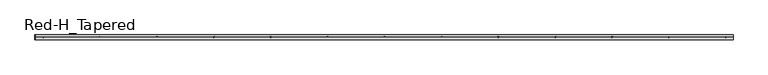
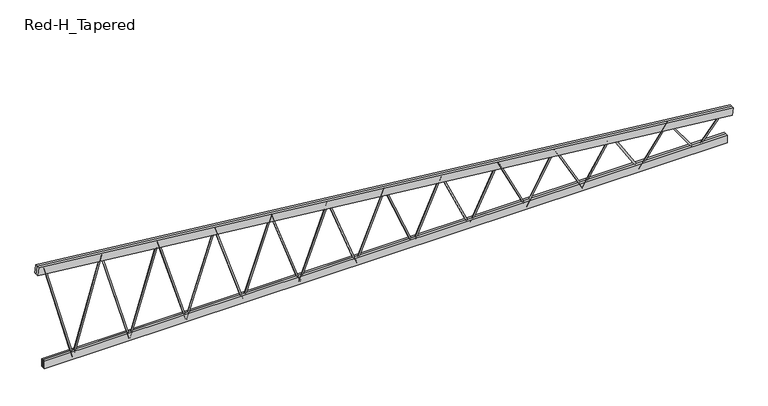
"""IFC4 building model written with IfcOpenShell, lengths in millimetres: beam geometry, Construction_Frames_RedBuilt_Openweb_Red-H_Tapered : Red-H_Tapered."""

from ifc_helpers import new_model, si_unit, point, frame, origin, origin_2d, place, context, project, spatial, polyline, circle_curve, trimmed, segment, composite_curve, outline, extrude, source, transform, mapped, element, save


def red_h_tapered_06906efe(model_context):
    return source(origin(), model_context, "Body", "SweptSolid", [
        extrude(outline(composite_curve([segment(trimmed(circle_curve(origin_2d(), 12.7), [point((0.0, -12.7))], [point((0.0, 12.7))], False, "CARTESIAN"), True, "CONTINUOUS"), segment(trimmed(circle_curve(origin_2d(), 12.7), [point((0.0, 12.7))], [point((0.0, -12.7))], False, "CARTESIAN"), True, "CONTINUOUS")], self_intersect=False)), frame((-491.6619792, 0.0, -367.0101562), z_axis=(-0.3557899484790522, 0.0, 0.9345659487490829), x_axis=(0.0, -1.0, 0.0)), (0.0, 0.0, 1.0), 1381.888334),
        extrude(outline(composite_curve([segment(trimmed(circle_curve(origin_2d(), 12.7), [point((0.0, 12.7))], [point((0.0, -12.6999999))], False, "CARTESIAN"), True, "CONTINUOUS"), segment(trimmed(circle_curve(origin_2d(), 12.7), [point((0.0, -12.6999999))], [point((0.0, 12.7))], False, "CARTESIAN"), True, "CONTINUOUS")], self_intersect=False)), frame((-1474.9859375, 0.0, -367.0101562), z_axis=(0.35578994847905304, 0.0, 0.9345659487490826), x_axis=(0.0, -1.0, 0.0)), (0.0, 0.0, 1.0), 1381.888334),
        extrude(outline(composite_curve([segment(trimmed(circle_curve(origin_2d(), 12.7), [point((0.0, -12.7))], [point((0.0, 12.6999999))], False, "CARTESIAN"), True, "CONTINUOUS"), segment(trimmed(circle_curve(origin_2d(), 12.7), [point((0.0, 12.6999999))], [point((0.0, -12.7))], False, "CARTESIAN"), True, "CONTINUOUS")], self_intersect=False)), frame((-1474.9859375, 0.0, -367.0101562), z_axis=(-0.33293456473962296, 0.0, 0.9429499327120385), x_axis=(0.0, -1.0, 0.0)), (0.0, 0.0, 1.0), 1476.7525852),
        extrude(outline(composite_curve([segment(trimmed(circle_curve(origin_2d(), 12.7), [point((0.0, -12.7))], [point((0.0, 12.7))], False, "CARTESIAN"), True, "CONTINUOUS"), segment(trimmed(circle_curve(origin_2d(), 12.7), [point((0.0, 12.7))], [point((0.0, -12.7))], False, "CARTESIAN"), True, "CONTINUOUS")], self_intersect=False)), frame((-2458.3098958, 0.0, -367.0101562), z_axis=(0.3329345647396264, 0.0, 0.9429499327120373), x_axis=(0.0, -1.0, 0.0)), (0.0, 0.0, 1.0), 1476.7525852),
        extrude(outline(composite_curve([segment(trimmed(circle_curve(origin_2d(), 12.7), [point((0.0, 12.7))], [point((0.0, -12.7))], False, "CARTESIAN"), True, "CONTINUOUS"), segment(trimmed(circle_curve(origin_2d(), 12.7), [point((0.0, -12.7))], [point((0.0, 12.7))], False, "CARTESIAN"), True, "CONTINUOUS")], self_intersect=False)), frame((-2458.3098958, 0.0, -367.0101562), z_axis=(-0.3126852540143423, 0.0, 0.9498567954812905), x_axis=(0.0, -1.0, 0.0)), (0.0, 0.0, 1.0), 1572.3862026),
        extrude(outline(composite_curve([segment(trimmed(circle_curve(origin_2d(), 12.7), [point((0.0, -12.7))], [point((0.0, 12.7))], False, "CARTESIAN"), True, "CONTINUOUS"), segment(trimmed(circle_curve(origin_2d(), 12.7), [point((0.0, 12.7))], [point((0.0, -12.7))], False, "CARTESIAN"), True, "CONTINUOUS")], self_intersect=False)), frame((-3441.6338542, 0.0, -367.0101562), z_axis=(0.31268525401434183, 0.0, 0.9498567954812908), x_axis=(0.0, -1.0, 0.0)), (0.0, 0.0, 1.0), 1572.3862026),
        extrude(outline(composite_curve([segment(trimmed(circle_curve(origin_2d(), 12.7), [point((0.0, 12.7))], [point((0.0, -12.7))], False, "CARTESIAN"), True, "CONTINUOUS"), segment(trimmed(circle_curve(origin_2d(), 12.7), [point((0.0, -12.7))], [point((0.0, 12.7))], False, "CARTESIAN"), True, "CONTINUOUS")], self_intersect=False)), frame((-3441.6338542, 0.0, -367.0101562), z_axis=(-0.29464533787098635, 0.0, 0.9556066789589179), x_axis=(0.0, -1.0, 0.0)), (0.0, 0.0, 1.0), 1668.6569104),
        extrude(outline(composite_curve([segment(trimmed(circle_curve(origin_2d(), 12.7), [point((0.0, -12.7))], [point((0.0, 12.7))], False, "CARTESIAN"), True, "CONTINUOUS"), segment(trimmed(circle_curve(origin_2d(), 12.7), [point((0.0, 12.7))], [point((0.0, -12.7))], False, "CARTESIAN"), True, "CONTINUOUS")], self_intersect=False)), frame((-4424.9578125, 0.0, -367.0101562), z_axis=(0.2946453378709914, 0.0, 0.9556066789589164), x_axis=(0.0, -1.0, 0.0)), (0.0, 0.0, 1.0), 1668.6569104),
        extrude(outline(composite_curve([segment(trimmed(circle_curve(origin_2d(), 12.7), [point((0.0, 12.7))], [point((0.0, -12.7))], False, "CARTESIAN"), True, "CONTINUOUS"), segment(trimmed(circle_curve(origin_2d(), 12.7), [point((0.0, -12.7))], [point((0.0, 12.7))], False, "CARTESIAN"), True, "CONTINUOUS")], self_intersect=False)), frame((-4424.9578125, 0.0, -367.0101562), z_axis=(-0.2784893697457471, 0.0, 0.9604393114292109), x_axis=(0.0, -1.0, 0.0)), (0.0, 0.0, 1.0), 1765.46049),
        extrude(outline(composite_curve([segment(trimmed(circle_curve(origin_2d(), 12.7), [point((0.0, -12.7))], [point((0.0, 12.6999999))], False, "CARTESIAN"), True, "CONTINUOUS"), segment(trimmed(circle_curve(origin_2d(), 12.7), [point((0.0, 12.6999999))], [point((0.0, -12.7))], False, "CARTESIAN"), True, "CONTINUOUS")], self_intersect=False)), frame((-5408.2817708, 0.0, -367.0101562), z_axis=(0.27848936974574684, 0.0, 0.9604393114292109), x_axis=(0.0, -1.0, 0.0)), (0.0, 0.0, 1.0), 1765.46049),
        extrude(outline(composite_curve([segment(trimmed(circle_curve(origin_2d(), 12.7), [point((0.0, 12.7))], [point((0.0, -12.7000001))], False, "CARTESIAN"), True, "CONTINUOUS"), segment(trimmed(circle_curve(origin_2d(), 12.7), [point((0.0, -12.7000001))], [point((0.0, 12.7))], False, "CARTESIAN"), True, "CONTINUOUS")], self_intersect=False)), frame((-5408.2817708, 0.0, -367.0101562), z_axis=(-0.2639492777400816, 0.0, 0.9645365616608265), x_axis=(0.0, -1.0, 0.0)), (0.0, 0.0, 1.0), 1862.7138645),
        extrude(outline(composite_curve([segment(trimmed(circle_curve(origin_2d(), 12.7), [point((0.0, 12.7000001))], [point((0.0, -12.6999999))], False, "CARTESIAN"), True, "CONTINUOUS"), segment(trimmed(circle_curve(origin_2d(), 12.7), [point((0.0, -12.6999999))], [point((0.0, 12.7000001))], False, "CARTESIAN"), True, "CONTINUOUS")], self_intersect=False)), frame((5408.2817708, 0.0, -367.0101562), z_axis=(0.6439089672678159, 0.0, 0.7651021120557013), x_axis=(0.0, -1.0, 0.0)), (0.0, 0.0, 1.0), 763.5582111),
        extrude(outline(composite_curve([segment(trimmed(circle_curve(origin_2d(), 12.7), [point((0.0, -12.7))], [point((0.0, 12.7))], False, "CARTESIAN"), True, "CONTINUOUS"), segment(trimmed(circle_curve(origin_2d(), 12.7), [point((0.0, 12.7))], [point((0.0, -12.7))], False, "CARTESIAN"), True, "CONTINUOUS")], self_intersect=False)), frame((5408.2817708, 0.0, -367.0101562), z_axis=(-0.5829691057722732, 0.0, 0.8124943210355849), x_axis=(0.0, -1.0, 0.0)), (0.0, 0.0, 1.0), 843.3757026),
        extrude(outline(composite_curve([segment(trimmed(circle_curve(origin_2d(), 12.7), [point((0.0, 12.7000001))], [point((0.0, -12.7))], False, "CARTESIAN"), True, "CONTINUOUS"), segment(trimmed(circle_curve(origin_2d(), 12.7), [point((0.0, -12.7))], [point((0.0, 12.7000001))], False, "CARTESIAN"), True, "CONTINUOUS")], self_intersect=False)), frame((4424.9578125, 0.0, -367.0101562), z_axis=(0.5829691057722711, 0.0, 0.8124943210355865), x_axis=(0.0, -1.0, 0.0)), (0.0, 0.0, 1.0), 843.3757026),
        extrude(outline(composite_curve([segment(trimmed(circle_curve(origin_2d(), 12.7), [point((0.0, -12.7))], [point((0.0, 12.6999999))], False, "CARTESIAN"), True, "CONTINUOUS"), segment(trimmed(circle_curve(origin_2d(), 12.7), [point((0.0, 12.6999999))], [point((0.0, -12.7))], False, "CARTESIAN"), True, "CONTINUOUS")], self_intersect=False)), frame((4424.9578125, 0.0, -367.0101562), z_axis=(-0.5301846601927273, 0.0, 0.8478822006011933), x_axis=(0.0, -1.0, 0.0)), (0.0, 0.0, 1.0), 927.3410117),
        extrude(outline(composite_curve([segment(trimmed(circle_curve(origin_2d(), 12.7), [point((0.0, 12.7))], [point((0.0, -12.7))], False, "CARTESIAN"), True, "CONTINUOUS"), segment(trimmed(circle_curve(origin_2d(), 12.7), [point((0.0, -12.7))], [point((0.0, 12.7))], False, "CARTESIAN"), True, "CONTINUOUS")], self_intersect=False)), frame((3441.6338542, 0.0, -367.0101562), z_axis=(0.5301846601927259, 0.0, 0.8478822006011942), x_axis=(0.0, -1.0, 0.0)), (0.0, 0.0, 1.0), 927.3410117),
        extrude(outline(composite_curve([segment(trimmed(circle_curve(origin_2d(), 12.7), [point((0.0, -12.7))], [point((0.0, 12.7))], False, "CARTESIAN"), True, "CONTINUOUS"), segment(trimmed(circle_curve(origin_2d(), 12.7), [point((0.0, 12.7))], [point((0.0, -12.7))], False, "CARTESIAN"), True, "CONTINUOUS")], self_intersect=False)), frame((3441.6338542, 0.0, -367.0101562), z_axis=(-0.48467074935534044, 0.0, 0.874696670120181), x_axis=(0.0, -1.0, 0.0)), (0.0, 0.0, 1.0), 1014.4246993),
        extrude(outline(composite_curve([segment(trimmed(circle_curve(origin_2d(), 12.7), [point((0.0, 12.7))], [point((0.0, -12.7))], False, "CARTESIAN"), True, "CONTINUOUS"), segment(trimmed(circle_curve(origin_2d(), 12.7), [point((0.0, -12.7))], [point((0.0, 12.7))], False, "CARTESIAN"), True, "CONTINUOUS")], self_intersect=False)), frame((2458.3098958, 0.0, -367.0101562), z_axis=(0.48467074935534116, 0.0, 0.8746966701201807), x_axis=(0.0, -1.0, 0.0)), (0.0, 0.0, 1.0), 1014.4246993),
        extrude(outline(composite_curve([segment(trimmed(circle_curve(origin_2d(), 12.7), [point((0.0, -12.7))], [point((0.0, 12.7))], False, "CARTESIAN"), True, "CONTINUOUS"), segment(trimmed(circle_curve(origin_2d(), 12.7), [point((0.0, 12.7))], [point((0.0, -12.7))], False, "CARTESIAN"), True, "CONTINUOUS")], self_intersect=False)), frame((2458.3098958, 0.0, -367.0101562), z_axis=(-0.44539077547183614, 0.0, 0.8953362815861963), x_axis=(0.0, -1.0, 0.0)), (0.0, 0.0, 1.0), 1103.8890032),
        extrude(outline(composite_curve([segment(trimmed(circle_curve(origin_2d(), 12.7), [point((0.0, 12.7))], [point((0.0, -12.7))], False, "CARTESIAN"), True, "CONTINUOUS"), segment(trimmed(circle_curve(origin_2d(), 12.7), [point((0.0, -12.7))], [point((0.0, 12.7))], False, "CARTESIAN"), True, "CONTINUOUS")], self_intersect=False)), frame((1474.9859375, 0.0, -367.0101562), z_axis=(0.4453907754718395, 0.0, 0.8953362815861946), x_axis=(0.0, -1.0, 0.0)), (0.0, 0.0, 1.0), 1103.8890032),
        extrude(outline(composite_curve([segment(trimmed(circle_curve(origin_2d(), 12.7), [point((0.0, -12.7))], [point((0.0, 12.7))], False, "CARTESIAN"), True, "CONTINUOUS"), segment(trimmed(circle_curve(origin_2d(), 12.7), [point((0.0, 12.7))], [point((0.0, -12.7))], False, "CARTESIAN"), True, "CONTINUOUS")], self_intersect=False)), frame((1474.9859375, 0.0, -367.0101562), z_axis=(-0.41136395902525347, 0.0, 0.9114711697114011), x_axis=(0.0, -1.0, 0.0)), (0.0, 0.0, 1.0), 1195.1994539),
        extrude(outline(composite_curve([segment(trimmed(circle_curve(origin_2d(), 12.7), [point((0.0, 12.7))], [point((0.0, -12.7))], False, "CARTESIAN"), True, "CONTINUOUS"), segment(trimmed(circle_curve(origin_2d(), 12.7), [point((0.0, -12.7))], [point((0.0, 12.7))], False, "CARTESIAN"), True, "CONTINUOUS")], self_intersect=False)), frame((491.6619792, 0.0, -367.0101562), z_axis=(0.41136395902525497, 0.0, 0.9114711697114004), x_axis=(0.0, -1.0, 0.0)), (0.0, 0.0, 1.0), 1195.1994539),
        extrude(outline(composite_curve([segment(trimmed(circle_curve(origin_2d(), 12.7), [point((0.0, -12.7))], [point((0.0, 12.7))], False, "CARTESIAN"), True, "CONTINUOUS"), segment(trimmed(circle_curve(origin_2d(), 12.7), [point((0.0, 12.7))], [point((0.0, -12.7))], False, "CARTESIAN"), True, "CONTINUOUS")], self_intersect=False)), frame((491.6619792, 0.0, -367.0101562), z_axis=(-0.3817359681353616, 0.0, 0.9242714161066317), x_axis=(0.0, -1.0, 0.0)), (0.0, 0.0, 1.0), 1287.9634622),
        extrude(outline(composite_curve([segment(trimmed(circle_curve(origin_2d(), 12.7), [point((0.0, 12.7))], [point((0.0, -12.7))], False, "CARTESIAN"), True, "CONTINUOUS"), segment(trimmed(circle_curve(origin_2d(), 12.7), [point((0.0, -12.7))], [point((0.0, 12.7))], False, "CARTESIAN"), True, "CONTINUOUS")], self_intersect=False)), frame((-491.6619792, 0.0, -367.0101562), z_axis=(0.38173596813532995, 0.0, 0.9242714161066448), x_axis=(0.0, -1.0, 0.0)), (0.0, 0.0, 1.0), 1287.9634622),
        extrude(outline(polyline([(-5925.34375, -41.275), (-5925.34375, -3.175), (5925.34375, -3.175), (5925.34375, -41.275), (-5925.34375, -41.275)])), frame((0.0, 0.0, -386.0601562), z_axis=(0.0, 0.0, 1.0), x_axis=(1.0, 0.0, 0.0)), (0.0, 0.0, 1.0), 139.7),
        extrude(outline(polyline([(-5925.34375, 3.175), (-5925.34375, 41.275), (5925.34375, 41.275), (5925.34375, 3.175), (-5925.34375, 3.175)])), frame((0.0, 0.0, -386.0601562), z_axis=(0.0, 0.0, 1.0), x_axis=(1.0, 0.0, 0.0)), (0.0, 0.0, 1.0), 139.7),
        extrude(outline(polyline([(0.0, -38.1), (0.0, 0.0), (12121.9438686, 0.0), (12121.9438686, -38.1), (0.0, -38.1)])), frame((-6041.7262958, -3.175, 1367.3241631), z_axis=(0.10581636195546908, 0.0, 0.9943856885245831), x_axis=(0.9943856885245831, 0.0, -0.10581636195546908)), (0.0, 0.0, 1.0), 139.7),
        extrude(outline(polyline([(0.0, -38.1), (0.0, 0.0), (12121.9438686, 0.0), (12121.9438686, -38.1), (0.0, -38.1)])), frame((-6041.7262958, 41.275, 1367.3241631), z_axis=(0.10581636195546908, 0.0, 0.9943856885245831), x_axis=(0.9943856885245831, 0.0, -0.10581636195546908)), (0.0, 0.0, 1.0), 139.7),
    ])


if __name__ == "__main__":
    model = new_model("IFC4")
    model_context = context("Model", 3, world=origin())
    ifc_project = project(units=[si_unit("LENGTHUNIT", "METRE", prefix="MILLI")], contexts=[model_context])
    site = spatial("IfcSite", under=ifc_project)
    building = spatial("IfcBuilding", under=site)
    placement = place(None, origin())
    red_h_tapered_shape = red_h_tapered_06906efe(model_context)
    element("IfcBeam", 1, ObjectType="Construction_Frames_RedBuilt_Openweb_Red-H_Tapered : Red-H_Tapered", at=placement, inside=building, context=model_context, shape_type="MappedRepresentation", body=[
        mapped(red_h_tapered_shape, transform((0.0, 0.0, 0.0), x_axis=(1.0, 0.0, 0.0), y_axis=(0.0, 1.0, 0.0), z_axis=(0.0, 0.0, 1.0))),
    ])
    save(model, "model.ifc")

# Revit data of these elements
# Type "Construction_Frames_RedBuilt_Openweb_Red-H_Tapered : Red-H_Tapered"
#   Youtube clip = ""
#   Weight Net (Kg) = "0"
#   Webs = "Up to 2\" diameter tubular steel"
#   Uniformat II Description = ""
#   Uniformat II Code = ""
#   Uniclass 2015 Name = "Softwood trusses"
#   Uniclass 2015 Code = "Pr_20_85_90_81"
#   Uniclass 2.0 Description = "Structural Framing Systems"
#   Uniclass 2.0 Code = "SS-15-10-75"
#   Uniclass 1.4 Description = "Trusses"
#   Uniclass 1.4 Code = "L3523"
#   UNSPSC Code = "30103606"
#   Technical description = "http://www.redbuilt.com/reference/literature-and-other-resources"
#   Region South America = "None"
#   Region Oceania = "None"
#   Region North America = "US"
#   Region Middle East = "None"
#   Region Europe = "None"
#   Region Asia = "None"
#   Region Antarctica = "None"
#   Region Africa = "None"
#   QR code = "http://bimobject.com/redbuilt/product/redbuilt-0003"
#   Product url = "http://www.redbuilt.com/products/default.aspx?id=2"
#   Product group = "Wood Trusses"
#   Product family = "Construction"
#   Product data url = "https://bimobject.com/redbuilt/product/redbuilt-0003"
#   Product certification = ""
#   Product SKU = "redbuilt-0003"
#   Product Page URL = "http://www.redbuilt.com/commercial-systems/red-m-red-h-open-web-trusses"
#   Product Guid = "2c5793f2-6ffb-4665-b825-cf90c048e711"
#   Product Documentation Link = "http://www.redbuilt.com/documents/OW_Guide_2017_07_LowRes_wLinks.pdf"
#   OmniClass Description = "Wood Trusses"
#   OmniClass Code = "23-13 35 19 13 17"
#   NBS Reference Description = ""
#   NBS Reference Code = ""
#   Material secondary = "Steel"
#   Material main = "Wood"
#   Masterformat 2014 Description = "Metal-Web Wood Joists"
#   Masterformat 2014 Code = "06 17 36"
#   Manufacturer name = "RedBuilt"
#   Manufacturer country = "United States"
#   Installation instructions = "http://www.redbuilt.com/documents/Installation_Sheets_Open-Web.pdf"
#   IFC Classification = ""
#   EAN code = ""
#   Design country = "United States"
#   Product Information = "http://redbuilt.com/products/default.aspx?id=2"
#   Model = "Red-H-Tapered"
#   Manufacturer URL = "http://redbuilt.com/"
#   Manufacturer = "RedBuilt™"
#   Description = "Open Web Truss"
#   Date of publishing = "8/17/2010"
#   Contact us = "http://redbuilt.com/contact/"
#   Chords = "Double 1½\" x 5½\" MSR lumber"
#   COBIe Type Category = ""
#   Brand url = "http://www.redbuilt.com"
#   BIMobject main category code = "construction"
#   BIMobject main category = "Construction"
#   BIMobject category code = "construction-frames-trusses"
#   BIMobject category = "Frames & Trusses"
#   Web Radius = 0' - 0 1/2"
#   Web Layout Offset Start [instance default] = 0' - 5"
#   Web Layout Offset End [instance default] = 0' - 5"
#   Web Diameter = 0' - 1"
#   TotalLength [instance default] = 20' - 0"
#   Span Minimum = 4' - 0"
#   Span Maximum = 70' - 0"
#   Span Limit [instance default] = 20' - 0"
#   Nominal width = 0' - 0"
#   Nominal height = 0' - 0"
#   Inner Depth Top [instance default] = 0' - 2.76372"
#   Depth Start [instance default] = 6' - 0"
#   Top Chord Length [instance default] = 20' - 1.19701"
#   TC Extension Start Aux [instance default] = 0' - 0"
#   TC Extension End Aux [instance default] = 0' - 0"
#   T-B Chord Length Difference L [instance default] = 0' - 4"
#   T-B Chord Length Difference [instance default] = 0' - 4"
#   Height 2 [instance default] = 6' - 0"
#   Depth Minimum at Wall = 2' - 0"
#   Depth Maximum at Wall = 6' - 0"
#   Depth Lower End [instance default] = 2' - 0"
#   Depth Higher End [instance default] = 6' - 0"
#   Depth End [instance default] = 2' - 0"
#   Depth 2 [instance default] = 2' - 0"
#   Chord Width = 0' - 3 1/4"
#   Chord Thickness = 0' - 1 1/2"
#   Chord Depth = 0' - 5 1/2"
#   Offset Start [instance default] = 0' - 0"
#   TC Extension Start [instance default] = 0' - 0"
#   End Panel = 0' - 5"
#   Offset End [instance default] = 0' - 0"
#   TC Extension End [instance default] = 0' - 0"
#   Length [instance default] = 20' - 0"
#   Angle [instance default] = 5.71059°
#   Span Limit Warning [instance default] = no
#   Edition number = 1
#   Top Bearing Start [instance default] = yes
#   Top Bearing End [instance default] = yes
#   Bottom Bearing Start [instance default] = no
#   Bottom Bearing End [instance default] = no
#   8 Panels [instance default] = yes
#   16 Panels [instance default] = no
#   12 Panels [instance default] = no
#   Web Material = RedBuilt-Steel, Galvanized
#   Clip Material = RedBuilt-Steel, Galvanized
#   Chords Material = RedBuilt-MSR
#   URL = ""
#   Assembly Code = ""
# Element 1 (IfcBeam, "Construction_Frames_RedBuilt_Openweb_Red-H_Tapered : Red-H_Tapered")
#   TotalLength = 39' - 6 9/16"
#   Span Limit = 39' - 6 9/16"
#   Inner Depth Top = 0' - 2.76553"
#   Top Chord Length = 39' - 9.24188"
#   Depth 2 = 4' - 2 1/2"
#   Angle = 6.0742°
#   8 Panels = no
#   12 Panels = yes
#   Materials on its faces: "RedBuilt-Steel, Galvanized", "RedBuilt-MSR"
# Materials
#   "RedBuilt-Steel, Galvanized": class "Metal", colour RGB 164 172 176, transparency 0, Manufacturer = "RedBuilt. LLC", Comments = "Openweb Metal Web", URL = "http://www.redbuilt.com/", Description = "Galvanized steel", Cost = 0
#   "RedBuilt-MSR": class "Wood", colour RGB 213 182 136, transparency 0, Manufacturer = "RedBuilt, LLC", URL = "http://www.redbuilt.com/", Cost = 0
